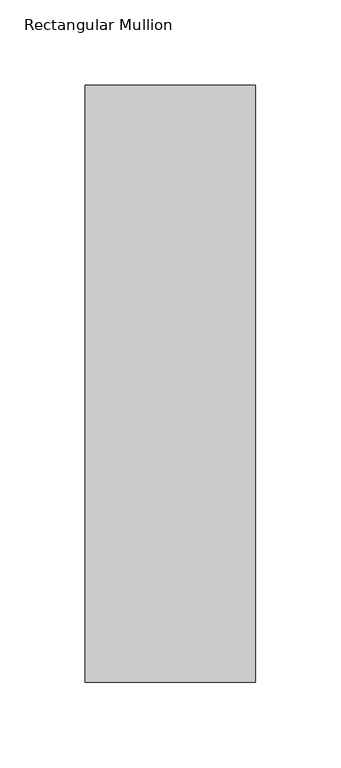
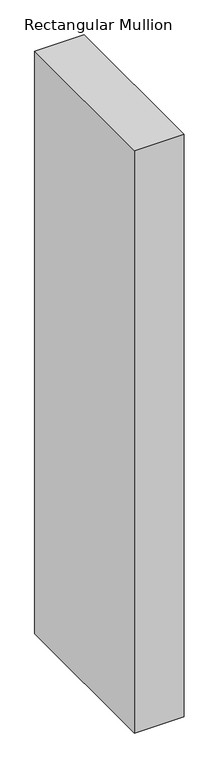
"""IFC4 building model written with IfcOpenShell, lengths in millimetres: member geometry, Rectangular Mullion : WWm-100x350-100mmOffset."""

from ifc_helpers import new_model, si_unit, frame, origin, place, context, project, spatial, polyline, outline, extrude, source, transform, mapped, element, save


def rectangular_mullion_9a6ec2c7(model_context):
    return source(origin(), model_context, "Body", "SweptSolid", [
        extrude(outline(polyline([(0.0, 175.0), (0.0, -175.0), (-100.0, -175.0), (-100.0, 175.0), (0.0, 175.0)])), frame((0.0, 0.0, -1245.7959447), z_axis=(0.0, 0.0, 1.0), x_axis=(1.0, 0.0, 0.0)), (0.0, 0.0, 1.0), 1245.7959447),
    ])


if __name__ == "__main__":
    model = new_model("IFC4")
    model_context = context("Model", 3, world=origin())
    ifc_project = project(units=[si_unit("LENGTHUNIT", "METRE", prefix="MILLI")], contexts=[model_context])
    site = spatial("IfcSite", under=ifc_project)
    building = spatial("IfcBuilding", under=site)
    placement = place(None, origin())
    rectangular_mullion_shape = rectangular_mullion_9a6ec2c7(model_context)
    element("IfcMember", 1, ObjectType="Rectangular Mullion : WWm-100x350-100mmOffset", at=placement, inside=building, context=model_context, shape_type="MappedRepresentation", body=[
        mapped(rectangular_mullion_shape, transform((0.0, 0.0, 0.0), x_axis=(1.0, 0.0, 0.0), y_axis=(0.0, 1.0, 0.0), z_axis=(0.0, 0.0, 1.0))),
    ])
    save(model, "model.ifc")

# Revit data of these elements
# Type "Rectangular Mullion : WWm-100x350-100mmOffset"
#   built-in parameter 1007304 = 1.14829 (stored number, unit not read)
#   built-in parameter 1007301 = 0.164042 (stored number, unit not read)
#   built-in parameter 1007300 = 0.164042 (stored number, unit not read)
# Element 1 (IfcMember, "Rectangular Mullion : WWm-100x350-100mmOffset")
#   Materials on its faces: "WW-EC-RGB-Mullion"
# Materials
#   "WW-EC-RGB-Mullion": class "Generic", colour RGB 255 255 255, transparency 0, Comments = "If region requests black mullions, switch asset color to RGB 25-25-25", Description = "Generic Color", Cost = 0
